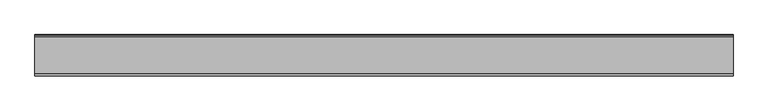
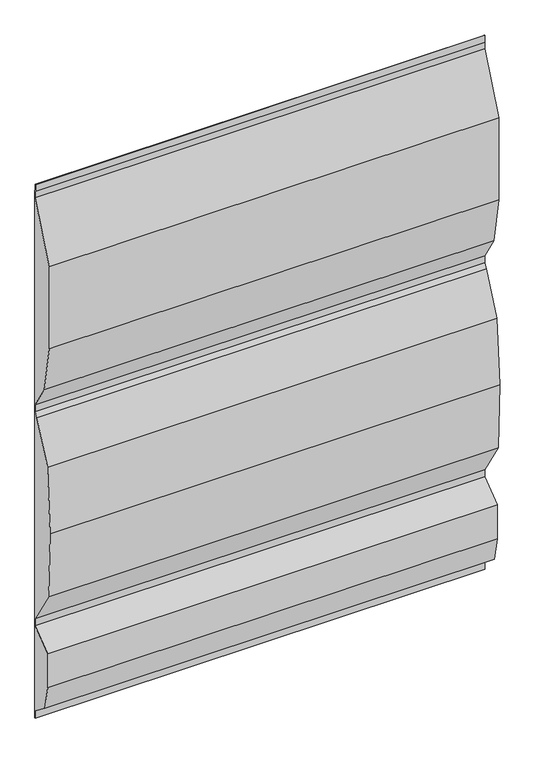
"""IFC4 building model written with IfcOpenShell, lengths in millimetres: proxy geometry, Generic Models 7:Generic Models 1:337419:Generic Models 1:337419 : Generic Models 7:Generic Models 1:337419:14 : Generic Models 7:Generic Models 1:337419:Generic Models 1:337419 : Generic Models 7:Generic Models 1:337419:301336."""

from ifc_helpers import new_model, si_unit, frame, origin, place, context, project, spatial, polyline, outline, extrude, source, transform, mapped, element, save


def generic_models_c1fb525a(model_context):
    return source(origin(), model_context, "Body", "SweptSolid", [
        extrude(outline(polyline([(-536554.1163358, 2617.9858565), (-536554.1163358, 2538.618119), (-536557.2913358, 2538.618119), (-536557.2913358, 2620.3783906), (-536743.4099128, 2760.6287981), (-536796.2655215, 3028.8889055), (-536796.2655215, 3421.101974), (-536557.2913358, 3598.4656655), (-536557.2913358, 3677.840625), (-536811.2913358, 4084.3255954), (-536841.9563951, 4820.287017), (-536790.5737765, 5555.0926964), (-536591.6998949, 6001.7707479), (-536557.2913358, 6049.5656655), (-536557.2913358, 6126.1625), (-536731.1813042, 6404.4446207), (-536823.8052422, 6929.7410761), (-536823.8052422, 7869.5410761), (-536557.2913358, 8500.6644623), (-536557.2913358, 8580.040625), (-536565.2288841, 8580.040625), (-536565.2288841, 8656.2497433), (-536561.1796979, 8656.2497433), (-536561.1796979, 8581.7240819), (-536554.1163358, 8581.7240819), (-536554.1163358, 2617.9858565)])), frame((591306.0367242, 0.0, 0.0), z_axis=(1.0, 0.0, 0.0), x_axis=(0.0, 1.0, 0.0)), (0.0, 0.0, 1.0), 4876.8),
    ])


if __name__ == "__main__":
    model = new_model("IFC4")
    model_context = context("Model", 3, world=origin())
    ifc_project = project(units=[si_unit("LENGTHUNIT", "METRE", prefix="MILLI")], contexts=[model_context])
    site = spatial("IfcSite", under=ifc_project)
    building = spatial("IfcBuilding", under=site)
    placement = place(None, origin())
    generic_models_shape = generic_models_c1fb525a(model_context)
    element("IfcBuildingElementProxy", 1, Name="Generic Models 7:Generic Models 1:337419:Generic Models 1:337419 : Generic Models 7:Generic Models 1:337419:14 : Generic Models 7:Generic Models 1:337419:Generic Models 1:337419 : Generic Models 7:Generic Models 1:337419:301336", ObjectType="Generic Models 7:Generic Models 1:337419:Generic Models 1:337419 : Generic Models 7:Generic Models 1:337419:14 : Generic Models 7:Generic Models 1:337419:Generic Models 1:337419 : Generic Models 7:Generic Models 1:337419:301336", at=placement, inside=building, context=model_context, shape_type="MappedRepresentation", body=[
        mapped(generic_models_shape, transform((0.0, 0.0, 0.0), x_axis=(1.0, 0.0, 0.0), y_axis=(0.0, 1.0, 0.0), z_axis=(0.0, 0.0, 1.0))),
    ])
    save(model, "model.ifc")

# Revit data of these elements
# Type "Generic Models 7:Generic Models 1:337419:Generic Models 1:337419 : Generic Models 7:Generic Models 1:337419:14 : Generic Models 7:Generic Models 1:337419:Generic Models 1:337419 : Generic Models 7:Generic Models 1:337419:301336"
#   NameOverride = "Generic Models 7:Generic Models 1:337419:Generic Models 1:337419 : Generic Models 7:Generic Models 1:337419:301336"
#   ObjectTypeOverride = "Generic Models 1:337419 : Generic Models 7:Generic Models 1:337419"
#   Reference = "Generic Models 1"
#   Tag = "301336"
# Element 1 (IfcBuildingElementProxy, "Generic Models 7:Generic Models 1:337419:Generic Models 1:337419 : Generic Models 7:Generic Models 1:337419:14 : Generic Models 7:Generic Models 1:337419:Generic Models 1:337419 : Generic Models 7:Generic Models 1:337419:301336")
#   Materials on its faces: "CLASS A FIBERGLASS INSULATION WITH DURABLE VAPOR BARRIER (WHITE) LINE"
# Materials
#   "CLASS A FIBERGLASS INSULATION WITH DURABLE VAPOR BARRIER (WHITE) LINE": class "Unassigned", colour RGB 187 139 199, transparency 0, Cost = 0
